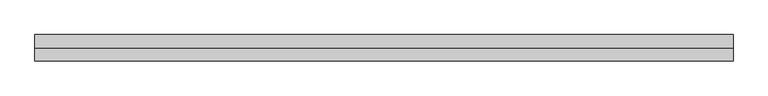
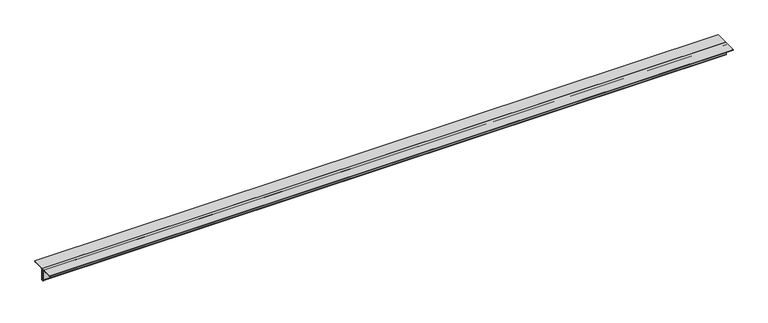
"""IFC4 building model written with IfcOpenShell, lengths in millimetres: member geometry, 0123_Steel Framing_2Ls-KSD3502 : H_SB_AR_S03_2Ls-130x130x12_HBR4."""

from ifc_helpers import new_model, si_unit, point, frame, frame_2d, origin, place, context, project, spatial, polyline, circle_curve, trimmed, segment, composite_curve, outline, extrude, source, transform, mapped, element, save


def member_5d4d22f8(model_context):
    return source(origin(), model_context, "Body", "SweptSolid", [
        extrude(outline(composite_curve([segment(polyline([(0.0, 36.4), (130.0, 36.4)]), True, "CONTINUOUS"), segment(trimmed(circle_curve(frame_2d((118.0, 36.4)), 12.0), [point((130.0, 36.4))], [point((118.0, 24.4))], False, "CARTESIAN"), True, "CONTINUOUS"), segment(polyline([(118.0, 24.4), (24.0, 24.4)]), True, "CONTINUOUS"), segment(trimmed(circle_curve(frame_2d((24.0, 12.4)), 12.0), [point((24.0, 24.4))], [point((12.0, 12.4))], True, "CARTESIAN"), True, "CONTINUOUS"), segment(polyline([(12.0, 12.4), (12.0, -81.6)]), True, "CONTINUOUS"), segment(trimmed(circle_curve(frame_2d((0.0, -81.6)), 12.0), [point((12.0, -81.6))], [point((0.0, -93.6))], False, "CARTESIAN"), True, "CONTINUOUS"), segment(polyline([(0.0, -93.6), (0.0, 36.4)]), True, "CONTINUOUS")], self_intersect=False)), frame((-3413.9998477, 0.0, 0.0), z_axis=(1.0, 0.0, 0.0), x_axis=(0.0, 1.0, 0.0)), (0.0, 0.0, 1.0), 6850.1941634),
        extrude(outline(composite_curve([segment(polyline([(0.0, 36.4), (0.0, -93.6)]), True, "CONTINUOUS"), segment(trimmed(circle_curve(frame_2d((0.0, -81.6)), 12.0), [point((0.0, -93.6))], [point((-12.0, -81.6))], False, "CARTESIAN"), True, "CONTINUOUS"), segment(polyline([(-12.0, -81.6), (-12.0, 12.4)]), True, "CONTINUOUS"), segment(trimmed(circle_curve(frame_2d((-24.0, 12.4)), 12.0), [point((-12.0, 12.4))], [point((-24.0, 24.4))], True, "CARTESIAN"), True, "CONTINUOUS"), segment(polyline([(-24.0, 24.4), (-118.0, 24.4)]), True, "CONTINUOUS"), segment(trimmed(circle_curve(frame_2d((-118.0, 36.4)), 12.0), [point((-118.0, 24.4))], [point((-130.0, 36.4))], False, "CARTESIAN"), True, "CONTINUOUS"), segment(polyline([(-130.0, 36.4), (0.0, 36.4)]), True, "CONTINUOUS")], self_intersect=False)), frame((-3413.9998477, 0.0, 0.0), z_axis=(1.0, 0.0, 0.0), x_axis=(0.0, 1.0, 0.0)), (0.0, 0.0, 1.0), 6850.1941634),
    ])


if __name__ == "__main__":
    model = new_model("IFC4")
    model_context = context("Model", 3, world=origin())
    ifc_project = project(units=[si_unit("LENGTHUNIT", "METRE", prefix="MILLI")], contexts=[model_context])
    site = spatial("IfcSite", under=ifc_project)
    building = spatial("IfcBuilding", under=site)
    placement = place(None, origin())
    member_shape = member_5d4d22f8(model_context)
    element("IfcMember", 1, ObjectType="0123_Steel Framing_2Ls-KSD3502 : H_SB_AR_S03_2Ls-130x130x12_HBR4", at=placement, inside=building, context=model_context, shape_type="MappedRepresentation", body=[
        mapped(member_shape, transform((0.0, 0.0, 0.0), x_axis=(1.0, 0.0, 0.0), y_axis=(0.0, 1.0, 0.0), z_axis=(0.0, 0.0, 1.0))),
    ])
    save(model, "model.ifc")

# Revit data of these elements
# Type "0123_Steel Framing_2Ls-KSD3502 : H_SB_AR_S03_2Ls-130x130x12_HBR4"
#   Type Mark = "HBR4"
#   Assembly Code = "B10"
#   Legs = "SLBB"
#   W = 8.97
#   Perimeter = 1.04 m²/m
#   Nominal Weight = 46.80 kgf/m
#   Length [instance default] = 1000 mm
#   Space = 0 mm
#   b = 130 mm
#   d = 130 mm
#   t = 12 mm
#   y = 36.4 mm
#   A = 0.005952 m²
#   Structural Material [instance default] = Steel ASTM A36
# Element 1 (IfcMember, "0123_Steel Framing_2Ls-KSD3502 : H_SB_AR_S03_2Ls-130x130x12_HBR4")
#   Materials on its faces: "Steel ASTM A36"
# Materials
#   "Steel ASTM A36": class "Metal", colour RGB 199 199 199, transparency 0, Description = "Structural steel, ASTM A36 Grade B, mill finish", Cost = 0
